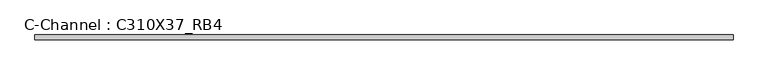
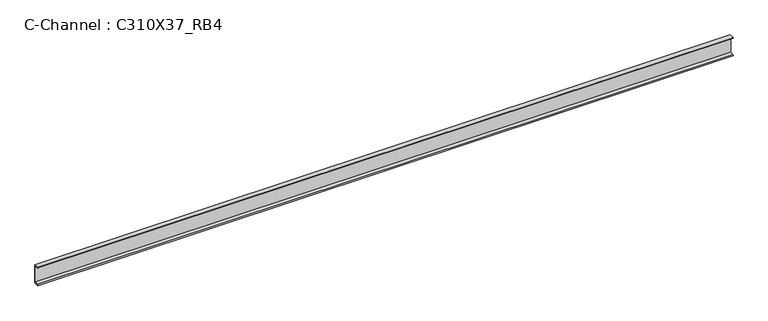
"""IFC4 building model written with IfcOpenShell, lengths in millimetres: beam geometry, C-Channel : C310X37_RB4."""

from ifc_helpers import new_model, si_unit, point, frame, frame_2d, origin, place, context, project, spatial, polyline, circle_curve, trimmed, segment, composite_curve, outline, extrude, source, transform, mapped, element, save


def c_channel_c310x37_rb4_f0f7eef8(model_context):
    return source(origin(), model_context, "Body", "SweptSolid", [
        extrude(outline(composite_curve([segment(polyline([(17.1196, 152.4), (17.1196, -152.4), (-60.3504, -152.4)]), True, "CONTINUOUS"), segment(trimmed(circle_curve(frame_2d((-47.625, -152.4)), 12.7254), [point((-60.3504, -152.4))], [point((-47.625, -139.6746))], False, "CARTESIAN"), True, "CONTINUOUS"), segment(polyline([(-47.625, -139.6746), (7.2898, -130.9769501), (7.2898, 130.9769501), (-47.625, 139.6746)]), True, "CONTINUOUS"), segment(trimmed(circle_curve(frame_2d((-47.625, 152.4)), 12.7254), [point((-47.625, 139.6746))], [point((-60.3504, 152.4))], False, "CARTESIAN"), True, "CONTINUOUS"), segment(polyline([(-60.3504, 152.4), (17.1196, 152.4)]), True, "CONTINUOUS")], self_intersect=False)), frame((-5530.0, 0.0, 0.0), z_axis=(1.0, 0.0, 0.0), x_axis=(0.0, 1.0, 0.0)), (0.0, 0.0, 1.0), 11060.0),
    ])


if __name__ == "__main__":
    model = new_model("IFC4")
    model_context = context("Model", 3, world=origin())
    ifc_project = project(units=[si_unit("LENGTHUNIT", "METRE", prefix="MILLI")], contexts=[model_context])
    site = spatial("IfcSite", under=ifc_project)
    building = spatial("IfcBuilding", under=site)
    placement = place(None, origin())
    c_channel_c310x37_rb4_shape = c_channel_c310x37_rb4_f0f7eef8(model_context)
    element("IfcBeam", 1, ObjectType="C-Channel : C310X37_RB4", at=placement, inside=building, context=model_context, shape_type="MappedRepresentation", body=[
        mapped(c_channel_c310x37_rb4_shape, transform((0.0, 0.0, 0.0), x_axis=(1.0, 0.0, 0.0), y_axis=(0.0, 1.0, 0.0), z_axis=(0.0, 0.0, 1.0))),
    ])
    save(model, "model.ifc")

# Revit data of these elements
# Type "C-Channel : C310X37_RB4"
#   Assembly Code = "B10"
#   W = 25
#   Length [instance default] = 1524 mm
#   bf = 77.47 mm
#   d = 304.8 mm
#   tf = 12.725 mm
#   tw = 9.83 mm
#   x = 17.12 mm
#   A = 0.00473547 m²
#   Structural Material [instance default] = Steel ASTM A36
# Element 1 (IfcBeam, "C-Channel : C310X37_RB4")
#   Structural Material = Steel ASTM A992
#   Materials on its faces: "Steel ASTM A992"
# Materials
#   "Steel ASTM A36": class "Metal", colour RGB 199 199 199, transparency 0, Description = "Structural steel, ASTM A36 Grade B, mill finish", Cost = 0
#   "Steel ASTM A992": class "Metal", colour RGB 199 199 199, transparency 0, Description = "Structural steel 50ksi", Cost = 0
